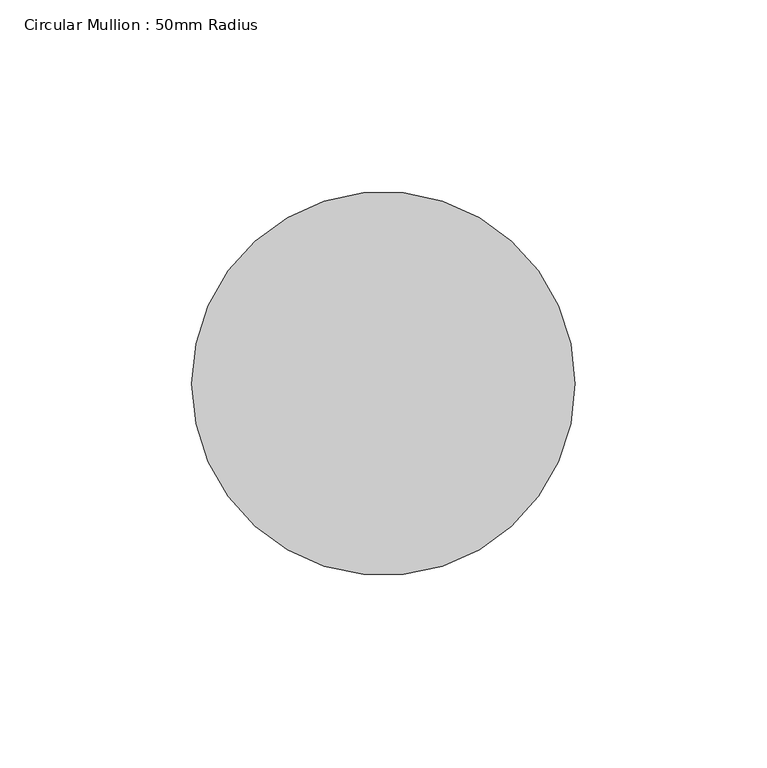
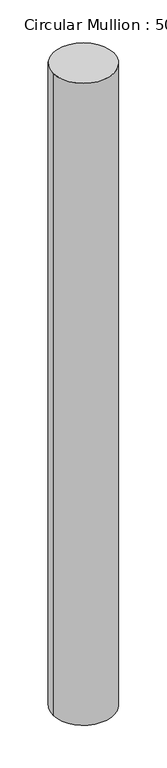
"""IFC4 building model written with IfcOpenShell, lengths in millimetres: member geometry, Circular Mullion : 50mm Radius."""

from ifc_helpers import new_model, si_unit, point, frame, origin, origin_2d, place, context, project, spatial, circle_curve, trimmed, segment, composite_curve, outline, extrude, source, transform, mapped, element, save


def circular_mullion_50mm_radius_9d1ad9a5(model_context):
    return source(origin(), model_context, "Body", "SweptSolid", [
        extrude(outline(composite_curve([segment(trimmed(circle_curve(origin_2d(), 50.0), [point((50.0, 0.0))], [point((-50.0, 0.0))], False, "CARTESIAN"), True, "CONTINUOUS"), segment(trimmed(circle_curve(origin_2d(), 50.0), [point((-50.0, 0.0))], [point((50.0, 0.0))], False, "CARTESIAN"), True, "CONTINUOUS")], self_intersect=False)), frame((0.0, 0.0, -1107.6005561), z_axis=(0.0, 0.0, 1.0), x_axis=(1.0, 0.0, 0.0)), (0.0, 0.0, 1.0), 1107.6005561),
    ])


if __name__ == "__main__":
    model = new_model("IFC4")
    model_context = context("Model", 3, world=origin())
    ifc_project = project(units=[si_unit("LENGTHUNIT", "METRE", prefix="MILLI")], contexts=[model_context])
    site = spatial("IfcSite", under=ifc_project)
    building = spatial("IfcBuilding", under=site)
    placement = place(None, origin())
    circular_mullion_50mm_radius_shape = circular_mullion_50mm_radius_9d1ad9a5(model_context)
    element("IfcMember", 1, ObjectType="Circular Mullion : 50mm Radius", at=placement, inside=building, context=model_context, shape_type="MappedRepresentation", body=[
        mapped(circular_mullion_50mm_radius_shape, transform((0.0, 0.0, 0.0), x_axis=(1.0, 0.0, 0.0), y_axis=(0.0, 1.0, 0.0), z_axis=(0.0, 0.0, 1.0))),
    ])
    save(model, "model.ifc")

# Revit data of these elements
# Type "Circular Mullion : 50mm Radius"
#   built-in parameter 1007350 = 0.164042 (stored number, unit not read)
# Element 1 (IfcMember, "Circular Mullion : 50mm Radius")
#   Materials on its faces: "Aluminium"
# Materials
#   "Aluminium": class "Metal", colour RGB 247 247 247, transparency 0, Description = "Aluminium 6061", Cost = 0
